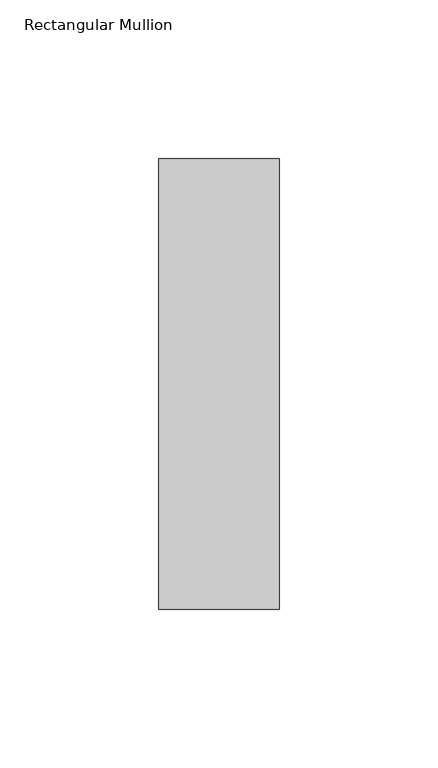
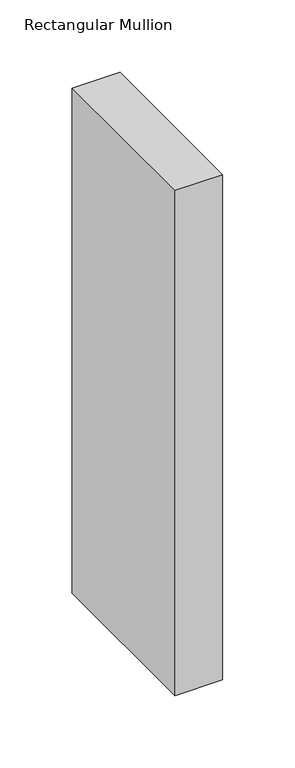
"""IFC4 building model written with IfcOpenShell, lengths in millimetres: member geometry, Rectangular Mullion : NLRS_21_CWM_hsb-regel 38x142_gen_rsf."""

from ifc_helpers import new_model, si_unit, frame, origin, place, context, project, spatial, polyline, outline, extrude, source, transform, mapped, element, save


def rectangular_mullion_afd5aca7(model_context):
    return source(origin(), model_context, "Body", "SweptSolid", [
        extrude(outline(polyline([(-38.0, -71.0), (-38.0, 71.0), (0.0, 71.0), (0.0, -71.0), (-38.0, -71.0)])), frame((0.0, 0.0, -426.0), z_axis=(0.0, 0.0, 1.0), x_axis=(1.0, 0.0, 0.0)), (0.0, 0.0, 1.0), 426.0),
    ])


if __name__ == "__main__":
    model = new_model("IFC4")
    model_context = context("Model", 3, world=origin())
    ifc_project = project(units=[si_unit("LENGTHUNIT", "METRE", prefix="MILLI")], contexts=[model_context])
    site = spatial("IfcSite", under=ifc_project)
    building = spatial("IfcBuilding", under=site)
    placement = place(None, origin())
    rectangular_mullion_shape = rectangular_mullion_afd5aca7(model_context)
    element("IfcMember", 1, ObjectType="Rectangular Mullion : NLRS_21_CWM_hsb-regel 38x142_gen_rsf", at=placement, inside=building, context=model_context, shape_type="MappedRepresentation", body=[
        mapped(rectangular_mullion_shape, transform((0.0, 0.0, 0.0), x_axis=(1.0, 0.0, 0.0), y_axis=(0.0, 1.0, 0.0), z_axis=(0.0, 0.0, 1.0))),
    ])
    save(model, "model.ifc")

# Revit data of these elements
# Type "Rectangular Mullion : NLRS_21_CWM_hsb-regel 38x142_gen_rsf"
#   Export Type to IFC As = "IfcWall"
#   Type IfcGUID = "07M7mRoiH1CR8m_RSKIwpF"
#   Assembly Code = "21.10"
#   built-in parameter 1007322 = 0.465879 (stored number, unit not read)
#   built-in parameter 1007321 = 0.062336 (stored number, unit not read)
#   built-in parameter 1007320 = 0.062336 (stored number, unit not read)
# Element 1 (IfcMember, "Rectangular Mullion : NLRS_21_CWM_hsb-regel 38x142_gen_rsf")
#   Materials on its faces: "NLRS_i2_hout naaldhout vuren_gen_rsf"
# Materials
#   "NLRS_i2_hout naaldhout vuren_gen_rsf": class "I - Hout", colour RGB 234 199 147, transparency 0, Keynote = "i2", Manufacturer = "Revit Standards Foundation", URL = "www.revitstandards.org", Description = "hout vuren", Cost = 0
